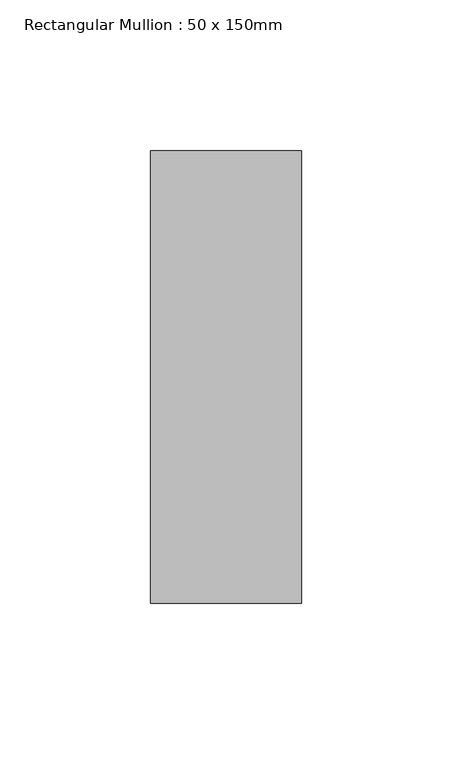
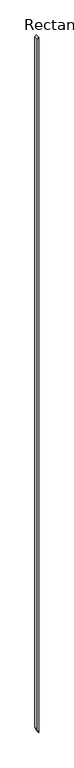
"""IFC4 building model written with IfcOpenShell, lengths in millimetres: member geometry, Rectangular Mullion : 50 x 150mm."""

from ifc_helpers import new_model, si_unit, frame, origin, place, context, project, spatial, polyline, outline, extrude, source, transform, mapped, element, save


def rectangular_mullion_50_x_150mm_d5752ba3(model_context):
    return source(origin(), model_context, "Body", "SweptSolid", [
        extrude(outline(polyline([(0.0, 0.0), (-53.1084457, -50.0), (-26319.8624924, -50.0), (-26470.1553886, 0.0), (0.0, 0.0)])), frame((0.0, -75.0, 0.0), z_axis=(0.0, 1.0, 0.0), x_axis=(0.0, 0.0, 1.0)), (0.0, 0.0, 1.0), 150.0),
    ])


if __name__ == "__main__":
    model = new_model("IFC4")
    model_context = context("Model", 3, world=origin())
    ifc_project = project(units=[si_unit("LENGTHUNIT", "METRE", prefix="MILLI")], contexts=[model_context])
    site = spatial("IfcSite", under=ifc_project)
    building = spatial("IfcBuilding", under=site)
    placement = place(None, origin())
    rectangular_mullion_50_x_150mm_shape = rectangular_mullion_50_x_150mm_d5752ba3(model_context)
    element("IfcMember", 1, ObjectType="Rectangular Mullion : 50 x 150mm", at=placement, inside=building, context=model_context, shape_type="MappedRepresentation", body=[
        mapped(rectangular_mullion_50_x_150mm_shape, transform((0.0, 0.0, 0.0), x_axis=(1.0, 0.0, 0.0), y_axis=(0.0, 1.0, 0.0), z_axis=(0.0, 0.0, 1.0))),
    ])
    save(model, "model.ifc")

# Revit data of these elements
# Type "Rectangular Mullion : 50 x 150mm"
#   built-in parameter 1007304 = 0.492126 (stored number, unit not read)
#   built-in parameter 1007301 = 0.082021 (stored number, unit not read)
#   built-in parameter 1007300 = 0.082021 (stored number, unit not read)
# Element 1 (IfcMember, "Rectangular Mullion : 50 x 150mm")
#   Materials on its faces: "Metal - Aluminium"
# Materials
#   "Metal - Aluminium": class "Metal", colour RGB 247 247 247, transparency 0
